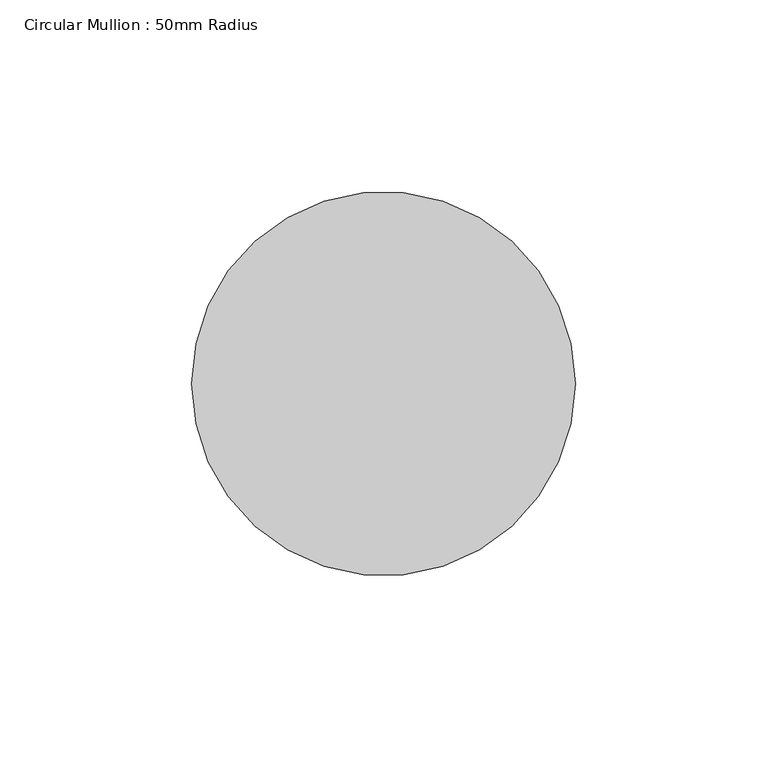
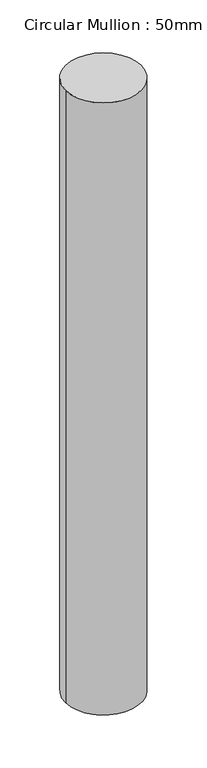
"""IFC4 building model written with IfcOpenShell, lengths in millimetres: member geometry, Circular Mullion : 50mm Radius."""

from ifc_helpers import new_model, si_unit, point, frame, origin, origin_2d, place, context, project, spatial, circle_curve, trimmed, segment, composite_curve, outline, extrude, source, transform, mapped, element, save


def circular_mullion_50mm_radius_bf28fd80(model_context):
    return source(origin(), model_context, "Body", "SweptSolid", [
        extrude(outline(composite_curve([segment(trimmed(circle_curve(origin_2d(), 50.0), [point((50.0, 0.0))], [point((-50.0, 0.0))], False, "CARTESIAN"), True, "CONTINUOUS"), segment(trimmed(circle_curve(origin_2d(), 50.0), [point((-50.0, 0.0))], [point((50.0, 0.0))], False, "CARTESIAN"), True, "CONTINUOUS")], self_intersect=False)), frame((0.0, 0.0, -855.495093), z_axis=(0.0, 0.0, 1.0), x_axis=(1.0, 0.0, 0.0)), (0.0, 0.0, 1.0), 855.495093),
    ])


if __name__ == "__main__":
    model = new_model("IFC4")
    model_context = context("Model", 3, world=origin())
    ifc_project = project(units=[si_unit("LENGTHUNIT", "METRE", prefix="MILLI")], contexts=[model_context])
    site = spatial("IfcSite", under=ifc_project)
    building = spatial("IfcBuilding", under=site)
    placement = place(None, origin())
    circular_mullion_50mm_radius_shape = circular_mullion_50mm_radius_bf28fd80(model_context)
    element("IfcMember", 1, ObjectType="Circular Mullion : 50mm Radius", at=placement, inside=building, context=model_context, shape_type="MappedRepresentation", body=[
        mapped(circular_mullion_50mm_radius_shape, transform((0.0, 0.0, 0.0), x_axis=(1.0, 0.0, 0.0), y_axis=(0.0, 1.0, 0.0), z_axis=(0.0, 0.0, 1.0))),
    ])
    save(model, "model.ifc")

# Revit data of these elements
# Type "Circular Mullion : 50mm Radius"
#   built-in parameter 1007350 = 0.164042 (stored number, unit not read)
# Element 1 (IfcMember, "Circular Mullion : 50mm Radius")
#   Materials on its faces: "Aluminium"
# Materials
#   "Aluminium": class "Metal", colour RGB 247 247 247, transparency 0, Description = "Aluminium 6061", Cost = 0
